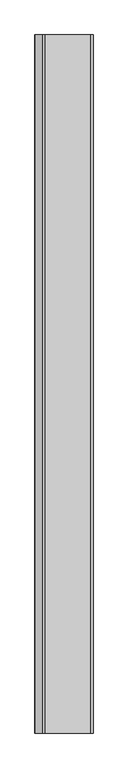
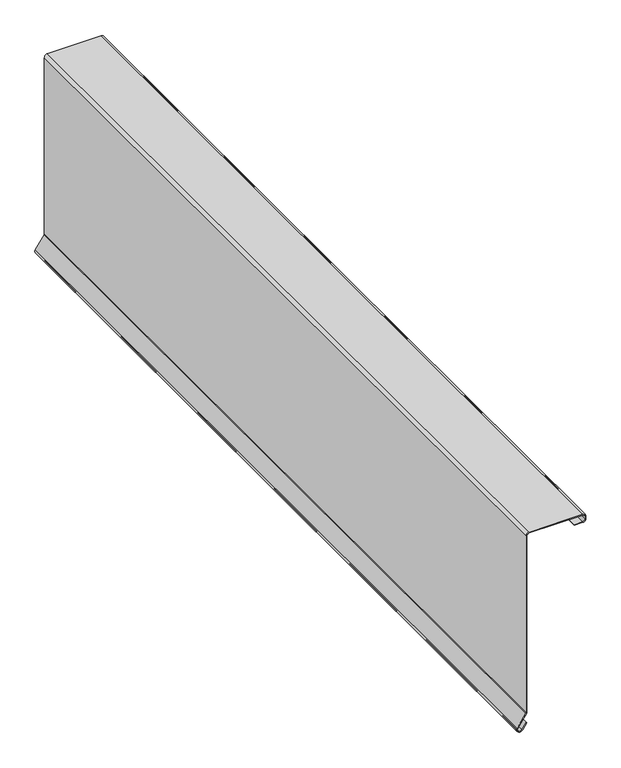
"""IFC4 building model written with IfcOpenShell, lengths in millimetres: proxy geometry, Flashing017 6369 : Flashing017 6369."""

from ifc_helpers import new_model, si_unit, point, frame, frame_2d, origin, place, context, project, spatial, polyline, circle_curve, trimmed, segment, composite_curve, outline, extrude, source, transform, mapped, element, save


def generic_models_3fb4e04b(model_context):
    return source(origin(), model_context, "Body", "SweptSolid", [
        extrude(outline(composite_curve([segment(trimmed(circle_curve(frame_2d((43730.1958627, 5305.6245867)), 5.08), [point((43727.2738024, 5309.7800606))], [point((43726.0843575, 5302.6409774))], True, "CARTESIAN"), True, "CONTINUOUS"), segment(polyline([(43726.0843575, 5302.6409774), (43727.3770366, 5300.8596259)]), True, "CONTINUOUS"), segment(trimmed(circle_curve(frame_2d((43731.4885418, 5303.8432352)), 5.08), [point((43727.3770366, 5300.8596259))], [point((43734.3956313, 5299.6772742))], True, "CARTESIAN"), True, "CONTINUOUS"), segment(polyline([(43734.3956313, 5299.6772742), (43764.6484819, 5320.788308)]), True, "CONTINUOUS"), segment(trimmed(circle_curve(frame_2d((43767.5555713, 5316.622347)), 5.08), [point((43764.6484819, 5320.788308))], [point((43767.5555713, 5321.702347))], False, "CARTESIAN"), True, "CONTINUOUS"), segment(polyline([(43767.5555713, 5321.702347), (44214.7845818, 5321.702347)]), True, "CONTINUOUS"), segment(trimmed(circle_curve(frame_2d((44214.7845818, 5326.782347)), 5.08), [point((44214.7845818, 5321.702347))], [point((44219.8645818, 5326.782347))], True, "CARTESIAN"), True, "CONTINUOUS"), segment(polyline([(44219.8645818, 5326.782347), (44219.8645818, 5456.122347)]), True, "CONTINUOUS"), segment(trimmed(circle_curve(frame_2d((44214.7845818, 5456.122347)), 5.08), [point((44219.8645818, 5456.122347))], [point((44214.7845818, 5461.202347))], True, "CARTESIAN"), True, "CONTINUOUS"), segment(polyline([(44214.7845818, 5461.202347), (44208.3781756, 5461.202347)]), True, "CONTINUOUS"), segment(trimmed(circle_curve(frame_2d((44208.3781756, 5456.122347)), 5.08), [point((44208.3781756, 5461.202347))], [point((44203.2981756, 5456.122347))], True, "CARTESIAN"), True, "CONTINUOUS"), segment(polyline([(44203.2981756, 5456.122347), (44203.2981756, 5434.8258822), (44201.2981756, 5434.8258822), (44201.2981756, 5456.122347)]), True, "CONTINUOUS"), segment(trimmed(circle_curve(frame_2d((44208.3781756, 5456.122347)), 7.08), [point((44201.2981756, 5456.122347))], [point((44208.3781756, 5463.202347))], False, "CARTESIAN"), True, "CONTINUOUS"), segment(polyline([(44208.3781756, 5463.202347), (44214.7845818, 5463.202347)]), True, "CONTINUOUS"), segment(trimmed(circle_curve(frame_2d((44214.7845818, 5456.122347)), 7.08), [point((44214.7845818, 5463.202347))], [point((44221.8645818, 5456.122347))], False, "CARTESIAN"), True, "CONTINUOUS"), segment(polyline([(44221.8645818, 5456.122347), (44221.8645818, 5326.782347)]), True, "CONTINUOUS"), segment(trimmed(circle_curve(frame_2d((44214.7845818, 5326.782347)), 7.08), [point((44221.8645818, 5326.782347))], [point((44214.7845818, 5319.702347))], False, "CARTESIAN"), True, "CONTINUOUS"), segment(polyline([(44214.7845818, 5319.702347), (43767.5555713, 5319.702347)]), True, "CONTINUOUS"), segment(trimmed(circle_curve(frame_2d((43767.5555713, 5316.622347)), 3.08), [point((43767.5555713, 5319.702347))], [point((43765.7930053, 5319.1481659))], True, "CARTESIAN"), True, "CONTINUOUS"), segment(polyline([(43765.7930053, 5319.1481659), (43735.5401547, 5298.0371321)]), True, "CONTINUOUS"), segment(trimmed(circle_curve(frame_2d((43731.4885418, 5303.8432352)), 7.08), [point((43735.5401547, 5298.0371321))], [point((43725.7583337, 5299.6849765))], False, "CARTESIAN"), True, "CONTINUOUS"), segment(polyline([(43725.7583337, 5299.6849765), (43724.4656546, 5301.466328)]), True, "CONTINUOUS"), segment(trimmed(circle_curve(frame_2d((43730.1958627, 5305.6245867)), 7.08), [point((43724.4656546, 5301.466328))], [point((43726.1233849, 5311.4160739))], False, "CARTESIAN"), True, "CONTINUOUS"), segment(polyline([(43726.1233849, 5311.4160739), (43740.7102581, 5321.6733213), (43741.8606756, 5320.037308), (43727.2738024, 5309.7800606)]), True, "CONTINUOUS")], self_intersect=False)), frame((0.0, -1052.8906574, 0.0), z_axis=(0.0, 1.0, 0.0), x_axis=(0.0, 0.0, 1.0)), (0.0, 0.0, 1.0), 2000.0),
    ])


if __name__ == "__main__":
    model = new_model("IFC4")
    model_context = context("Model", 3, world=origin())
    ifc_project = project(units=[si_unit("LENGTHUNIT", "METRE", prefix="MILLI")], contexts=[model_context])
    site = spatial("IfcSite", under=ifc_project)
    building = spatial("IfcBuilding", under=site)
    placement = place(None, origin())
    generic_models_shape = generic_models_3fb4e04b(model_context)
    element("IfcBuildingElementProxy", 1, Name="Flashing017 6369 : Flashing017 6369", ObjectType="Flashing017 6369 : Flashing017 6369", at=placement, inside=building, context=model_context, shape_type="MappedRepresentation", body=[
        mapped(generic_models_shape, transform((0.0, 0.0, 0.0), x_axis=(1.0, 0.0, 0.0), y_axis=(0.0, 1.0, 0.0), z_axis=(0.0, 0.0, 1.0))),
    ])
    save(model, "model.ifc")

# Revit data of these elements
# Type "Flashing017 6369 : Flashing017 6369"
#   NameOverride = "Flashing017"
# Element 1 (IfcBuildingElementProxy, "Flashing017 6369 : Flashing017 6369")
#   Materials on its faces: "HIGH EAVE FLASHING"
# Materials
#   "HIGH EAVE FLASHING": class "Unassigned", colour RGB 128 128 128, transparency 0
